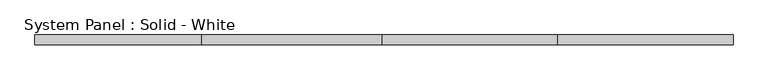
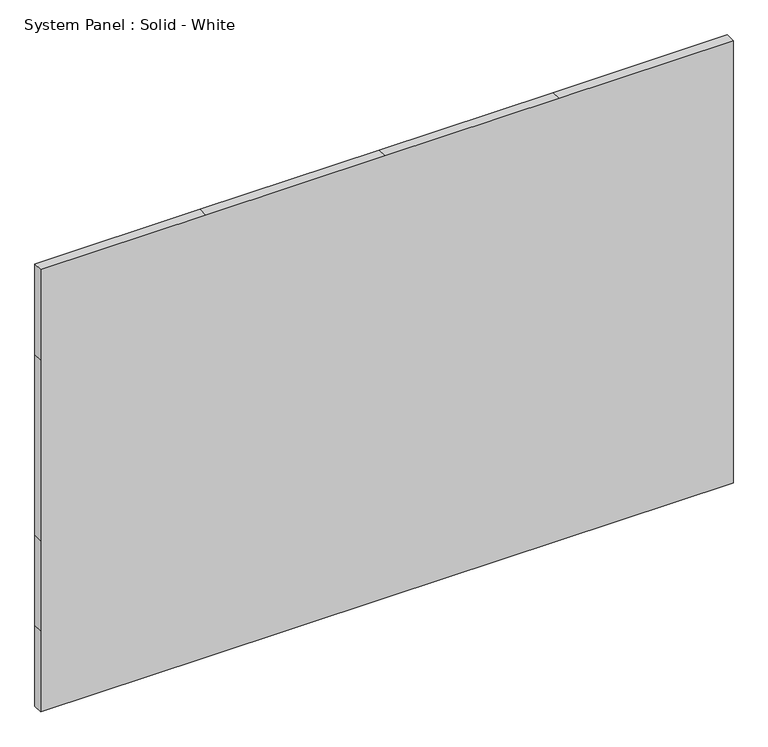
"""IFC4 building model written with IfcOpenShell, lengths in millimetres: plate geometry, System Panel : Solid - White."""

from ifc_helpers import new_model, si_unit, frame, origin, place, context, project, spatial, polyline, outline, extrude, source, transform, mapped, element, save


def system_panel_solid_white_958da58d(model_context):
    return source(origin(), model_context, "Body", "SweptSolid", [
        extrude(outline(polyline([(0.0, -2208.7972881), (0.0, -1154.0622881), (0.0, -11.3635593), (0.0, 1098.2827119), (0.0, 2208.7972881), (546.1, 2208.7972881), (1155.7, 2208.7972881), (2374.9, 2208.7972881), (2984.5, 2208.7972881), (2984.5, 1098.2827119), (2984.5, -11.3635593), (2984.5, -1154.0622881), (2984.5, -2208.7972881), (2374.9, -2208.7972881), (1155.7, -2208.7972881), (546.1, -2208.7972881), (0.0, -2208.7972881)])), frame((0.0, -44.45, 0.0), z_axis=(0.0, 1.0, 0.0), x_axis=(0.0, 0.0, 1.0)), (0.0, 0.0, 1.0), 63.5),
    ])


if __name__ == "__main__":
    model = new_model("IFC4")
    model_context = context("Model", 3, world=origin())
    ifc_project = project(units=[si_unit("LENGTHUNIT", "METRE", prefix="MILLI")], contexts=[model_context])
    site = spatial("IfcSite", under=ifc_project)
    building = spatial("IfcBuilding", under=site)
    placement = place(None, origin())
    system_panel_solid_white_shape = system_panel_solid_white_958da58d(model_context)
    element("IfcPlate", 1, ObjectType="System Panel : Solid - White", at=placement, inside=building, context=model_context, shape_type="MappedRepresentation", body=[
        mapped(system_panel_solid_white_shape, transform((0.0, 0.0, 0.0), x_axis=(1.0, 0.0, 0.0), y_axis=(0.0, 1.0, 0.0), z_axis=(0.0, 0.0, 1.0))),
    ])
    save(model, "model.ifc")

# Revit data of these elements
# Element 1 (IfcPlate, "System Panel : Solid - White")
#   Materials on its faces: "White Panel"
# Materials
#   "White Panel": class "Unassigned", colour RGB 255 255 255, transparency 0
